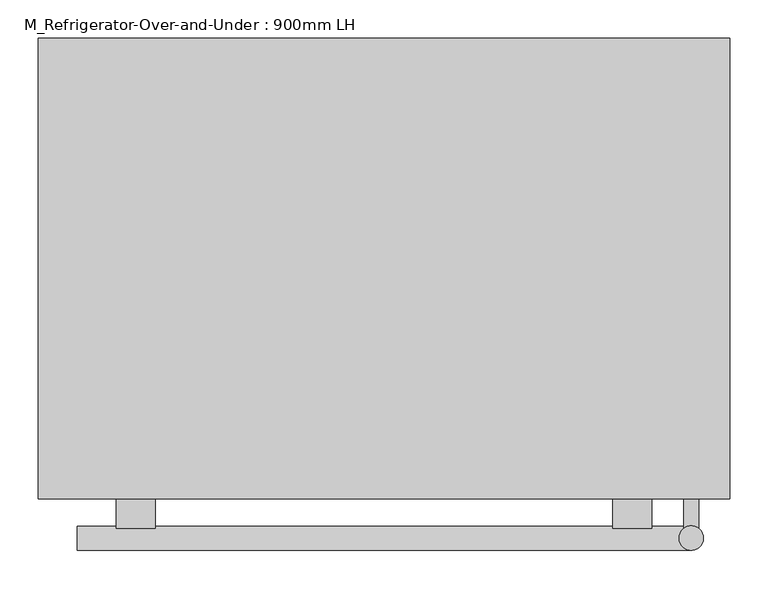
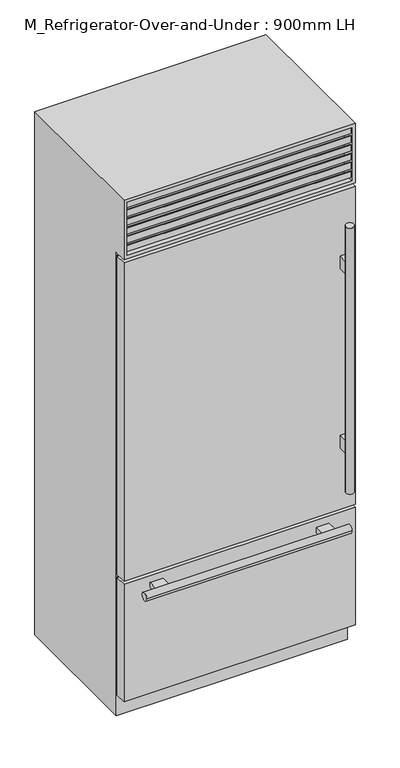
"""IFC4 building model written with IfcOpenShell, lengths in millimetres: proxy geometry, M_Refrigerator-Over-and-Under : 900mm LH."""

from ifc_helpers import new_model, si_unit, frame, origin, place, context, project, spatial, polyline, circle_curve, ellipse_curve, outline, extrude, faceted_brep, source, transform, mapped, element, save
from ifc_brep_helpers import plane_surface, cylinder_surface, advanced_brep


def m_refrigerator_over_and_under_900mm_lh_87200827(model_context):
    return source(origin(), model_context, "Body", "SolidModel", [
        extrude(outline(polyline([(-450.0, -655.55), (450.0, -655.55), (450.0, -700.0), (-450.0, -700.0), (-450.0, -655.55)])), frame((0.0, 0.0, 584.2), z_axis=(0.0, 0.0, 1.0), x_axis=(1.0, 0.0, 0.0)), (0.0, 0.0, 1.0), 1308.625),
        extrude(outline(polyline([(-450.0, -655.55), (450.0, -655.55), (450.0, -700.0), (-450.0, -700.0), (-450.0, -655.55)])), frame((0.0, 0.0, 88.9), z_axis=(0.0, 0.0, 1.0), x_axis=(1.0, 0.0, 0.0)), (0.0, 0.0, 1.0), 482.6),
        faceted_brep([(450.0, -700.0, 2150.0), (-450.0, -700.0, 2150.0), (-450.0, -700.0, 1905.525), (450.0, -700.0, 1905.525), (437.3, -700.0, 2137.3), (437.3, -700.0, 1918.225), (-437.3, -700.0, 1918.225), (-437.3, -700.0, 2137.3), (450.0, -100.0, 2150.0), (-450.0, -100.0, 2150.0), (-450.0, -100.0, 0.0), (-450.0, -649.2, 0.0), (-450.0, -649.2, 1905.525), (450.0, -649.2, 1905.525), (450.0, -649.2, 0.0), (450.0, -100.0, 0.0), (-437.3, -649.2, 2137.3), (437.3, -649.2, 2137.3), (-437.3, -649.2, 1918.225), (437.3, -649.2, 1918.225)], [[[0, 1, 2, 3], [4, 5, 6, 7]], [[1, 0, 8, 9]], [[2, 1, 9, 10, 11, 12]], [[3, 2, 12, 13]], [[8, 0, 3, 13, 14, 15]], [[4, 7, 16, 17]], [[7, 6, 18, 16]], [[6, 5, 19, 18]], [[5, 4, 17, 19]], [[15, 14, 11, 10]], [[9, 8, 15, 10]], [[17, 16, 18, 19]], [[11, 14, 13, 12]]]),
        extrude(outline(polyline([(-649.2, 1918.225), (-696.825, 1930.9860803), (-696.825, 1956.3860803), (-693.65, 1956.3860803), (-693.65, 1933.5368938), (-649.2, 1921.6265522), (-649.2, 1918.225)])), frame((-437.3, 0.0, 0.0), z_axis=(1.0, 0.0, 0.0), x_axis=(0.0, 1.0, 0.0)), (0.0, 0.0, 1.0), 874.6),
        extrude(outline(polyline([(-649.2, 1954.4077839), (-696.825, 1967.1688642), (-696.825, 1992.5688642), (-693.65, 1992.5688642), (-693.65, 1969.7196777), (-649.2, 1957.8093361), (-649.2, 1954.4077839)])), frame((-437.3, 0.0, 0.0), z_axis=(1.0, 0.0, 0.0), x_axis=(0.0, 1.0, 0.0)), (0.0, 0.0, 1.0), 874.6),
        extrude(outline(polyline([(-649.2, 1990.5905679), (-696.825, 2003.3516482), (-696.825, 2028.7516482), (-693.65, 2028.7516482), (-693.65, 2005.9024616), (-649.2, 1993.99212), (-649.2, 1990.5905679)])), frame((-437.3, 0.0, 0.0), z_axis=(1.0, 0.0, 0.0), x_axis=(0.0, 1.0, 0.0)), (0.0, 0.0, 1.0), 874.6),
        extrude(outline(polyline([(-649.2, 2026.7733518), (-696.825, 2039.5344321), (-696.825, 2064.9344321), (-693.65, 2064.9344321), (-693.65, 2042.0852456), (-649.2, 2030.174904), (-649.2, 2026.7733518)])), frame((-437.3, 0.0, 0.0), z_axis=(1.0, 0.0, 0.0), x_axis=(0.0, 1.0, 0.0)), (0.0, 0.0, 1.0), 874.6),
        extrude(outline(polyline([(-649.2, 2062.9561358), (-696.825, 2075.7172161), (-696.825, 2101.1172161), (-693.65, 2101.1172161), (-693.65, 2078.2680295), (-649.2, 2066.3576879), (-649.2, 2062.9561358)])), frame((-437.3, 0.0, 0.0), z_axis=(1.0, 0.0, 0.0), x_axis=(0.0, 1.0, 0.0)), (0.0, 0.0, 1.0), 874.6),
        extrude(outline(polyline([(-649.2, 2099.1389197), (-696.825, 2111.9), (-696.825, 2137.3), (-693.65, 2137.3), (-693.65, 2114.4508135), (-649.2, 2102.5404719), (-649.2, 2099.1389197)])), frame((-437.3, 0.0, 0.0), z_axis=(1.0, 0.0, 0.0), x_axis=(0.0, 1.0, 0.0)), (0.0, 0.0, 1.0), 874.6),
        advanced_brep(
        [(-443.65, -649.2, 565.15), (-443.65, -655.55, 565.15), (-443.65, -655.55, 95.25), (-443.65, -649.2, 95.25), (-446.825, -655.55, 568.325), (-446.825, -649.2, 568.325), (-446.825, -649.2, 92.075), (-446.825, -655.55, 92.075), (443.65, -655.55, 95.25), (443.65, -649.2, 95.25), (446.825, -649.2, 92.075), (446.825, -655.55, 92.075), (443.65, -655.55, 565.15), (443.65, -649.2, 565.15), (446.825, -649.2, 568.325), (446.825, -655.55, 568.325)],
        [
            (0, 1),
            (1, 2),
            (2, 3),
            (3, 0),
            (4, 5, ellipse_curve(frame((-446.825, -652.375, 568.325), z_axis=(-0.7071067811865475, 0.0, -0.7071067811865476), x_axis=(-0.7071067811865476, 0.0, 0.7071067811865475)), 4.4901281, 3.175)),
            (5, 6),
            (6, 7, ellipse_curve(frame((-446.825, -652.375, 92.075), z_axis=(-0.7071067811865475, 0.0, 0.7071067811865475), x_axis=(0.7071067811865474, 0.0, 0.7071067811865477)), 4.4901281, 3.175)),
            (7, 4),
            (2, 8),
            (8, 9),
            (9, 3),
            (6, 10),
            (10, 11, ellipse_curve(frame((446.825, -652.375, 92.075), z_axis=(-0.7071067811865475, 0.0, -0.7071067811865476), x_axis=(-0.7071067811865476, 0.0, 0.7071067811865474)), 4.4901281, 3.175)),
            (11, 7),
            (8, 12),
            (12, 13),
            (13, 9),
            (10, 14),
            (14, 15, ellipse_curve(frame((446.825, -652.375, 568.325), z_axis=(0.7071067811865476, 0.0, -0.7071067811865474), x_axis=(-0.7071067811865474, 0.0, -0.7071067811865477)), 4.4901281, 3.175)),
            (15, 11),
            (12, 1),
            (0, 13),
            (5, 14),
            (4, 15),
        ],
        [
            plane_surface(frame((-443.65, -655.55, 565.15), z_axis=(1.0, 0.0, 0.0), x_axis=(0.0, 0.0, -1.0))),
            cylinder_surface(frame((-446.825, -652.375, 571.5), z_axis=(0.0, 0.0, 1.0), x_axis=(0.0, -1.0, 0.0)), 3.175),
            plane_surface(frame((-443.65, -655.55, 95.25), z_axis=(0.0, 0.0, 1.0), x_axis=(1.0, 0.0, 0.0))),
            cylinder_surface(frame((-450.0, -652.375, 92.075), z_axis=(-1.0, 0.0, 0.0), x_axis=(0.0, -1.0, 0.0)), 3.175),
            plane_surface(frame((443.65, -655.55, 95.25), z_axis=(-1.0, 0.0, 0.0), x_axis=(0.0, 0.0, 1.0))),
            cylinder_surface(frame((446.825, -652.375, 88.9), z_axis=(0.0, 0.0, -1.0), x_axis=(0.0, -1.0, 0.0)), 3.175),
            plane_surface(frame((443.65, -655.55, 565.15), z_axis=(0.0, 0.0, -1.0), x_axis=(-1.0, 0.0, 0.0))),
            plane_surface(frame((443.65, -649.2, 565.15), z_axis=(0.0, 1.0, 0.0), x_axis=(-1.0, 0.0, 0.0))),
            cylinder_surface(frame((450.0, -652.375, 568.325), z_axis=(1.0, 0.0, 0.0), x_axis=(0.0, -1.0, 0.0)), 3.175),
            plane_surface(frame((446.825, -655.55, 568.325), z_axis=(0.0, -1.0, 0.0), x_axis=(-1.0, 0.0, 0.0))),
        ],
        [
            (0, [[1, 2, 3, 4]]),
            (1, [[5, 6, 7, 8]]),
            (2, [[-3, 9, 10, 11]]),
            (3, [[-7, 12, 13, 14]]),
            (4, [[-10, 15, 16, 17]]),
            (5, [[-13, 18, 19, 20]]),
            (6, [[-16, 21, -1, 22]]),
            (7, [[23, -18, -12, -6], [-11, -17, -22, -4]]),
            (8, [[-19, -23, -5, 24]]),
            (9, [[-14, -20, -24, -8], [-21, -15, -9, -2]]),
        ],
    ),
        advanced_brep(
        [(-443.65, -649.2, 1886.475), (-443.65, -655.55, 1886.475), (-443.65, -655.55, 590.55), (-443.65, -649.2, 590.55), (-446.825, -655.55, 1889.65), (-446.825, -649.2, 1889.65), (-446.825, -649.2, 587.375), (-446.825, -655.55, 587.375), (443.65, -655.55, 590.55), (443.65, -649.2, 590.55), (446.825, -649.2, 587.375), (446.825, -655.55, 587.375), (443.65, -655.55, 1886.475), (443.65, -649.2, 1886.475), (446.825, -649.2, 1889.65), (446.825, -655.55, 1889.65)],
        [
            (0, 1),
            (1, 2),
            (2, 3),
            (3, 0),
            (4, 5, ellipse_curve(frame((-446.825, -652.375, 1889.65), z_axis=(-0.7071067811865476, 0.0, -0.7071067811865475), x_axis=(-0.7071067811865475, 0.0, 0.7071067811865475)), 4.4901281, 3.175)),
            (5, 6),
            (6, 7, ellipse_curve(frame((-446.825, -652.375, 587.375), z_axis=(-0.7071067811865475, 0.0, 0.7071067811865476), x_axis=(0.7071067811865475, 0.0, 0.7071067811865475)), 4.4901281, 3.175)),
            (7, 4),
            (2, 8),
            (8, 9),
            (9, 3),
            (6, 10),
            (10, 11, ellipse_curve(frame((446.825, -652.375, 587.375), z_axis=(-0.7071067811865476, 0.0, -0.7071067811865475), x_axis=(-0.7071067811865475, 0.0, 0.7071067811865475)), 4.4901281, 3.175)),
            (11, 7),
            (8, 12),
            (12, 13),
            (13, 9),
            (10, 14),
            (14, 15, ellipse_curve(frame((446.825, -652.375, 1889.65), z_axis=(0.7071067811865474, 0.0, -0.7071067811865476), x_axis=(-0.7071067811865475, 0.0, -0.7071067811865476)), 4.4901281, 3.175)),
            (15, 11),
            (12, 1),
            (0, 13),
            (5, 14),
            (4, 15),
        ],
        [
            plane_surface(frame((-443.65, -655.55, 1886.475), z_axis=(1.0, 0.0, 0.0), x_axis=(0.0, 0.0, -1.0))),
            cylinder_surface(frame((-446.825, -652.375, 1892.825), z_axis=(0.0, 0.0, 1.0), x_axis=(0.0, -1.0, 0.0)), 3.175),
            plane_surface(frame((-443.65, -655.55, 590.55), z_axis=(0.0, 0.0, 1.0), x_axis=(1.0, 0.0, 0.0))),
            cylinder_surface(frame((-450.0, -652.375, 587.375), z_axis=(-1.0, 0.0, 0.0), x_axis=(0.0, -1.0, 0.0)), 3.175),
            plane_surface(frame((443.65, -655.55, 590.55), z_axis=(-1.0, 0.0, 0.0), x_axis=(0.0, 0.0, 1.0))),
            cylinder_surface(frame((446.825, -652.375, 584.2), z_axis=(0.0, 0.0, -1.0), x_axis=(0.0, -1.0, 0.0)), 3.175),
            plane_surface(frame((443.65, -655.55, 1886.475), z_axis=(0.0, 0.0, -1.0), x_axis=(-1.0, 0.0, 0.0))),
            plane_surface(frame((443.65, -649.2, 1886.475), z_axis=(0.0, 1.0, 0.0), x_axis=(-1.0, 0.0, 0.0))),
            cylinder_surface(frame((450.0, -652.375, 1889.65), z_axis=(1.0, 0.0, 0.0), x_axis=(0.0, -1.0, 0.0)), 3.175),
            plane_surface(frame((446.825, -655.55, 1889.65), z_axis=(0.0, -1.0, 0.0), x_axis=(-1.0, 0.0, 0.0))),
        ],
        [
            (0, [[1, 2, 3, 4]]),
            (1, [[5, 6, 7, 8]]),
            (2, [[-3, 9, 10, 11]]),
            (3, [[-7, 12, 13, 14]]),
            (4, [[-10, 15, 16, 17]]),
            (5, [[-13, 18, 19, 20]]),
            (6, [[-16, 21, -1, 22]]),
            (7, [[23, -18, -12, -6], [-11, -17, -22, -4]]),
            (8, [[-19, -23, -5, 24]]),
            (9, [[-14, -20, -24, -8], [-21, -15, -9, -2]]),
        ],
    ),
        advanced_brep(
        [(-297.6, -700.0, 542.925), (-297.6, -700.0, 523.875), (-348.4, -700.0, 523.875), (-348.4, -700.0, 542.925), (297.6, -700.0, 542.925), (348.4, -700.0, 542.925), (348.4, -700.0, 523.875), (297.6, -700.0, 523.875), (-297.6, -738.4741958, 542.925), (-297.6, -735.2991958, 533.4), (-297.6, -738.4741958, 523.875), (-348.4, -738.4741958, 523.875), (-348.4, -735.2991958, 533.4), (-348.4, -738.4741958, 542.925), (297.6, -738.4741958, 542.925), (348.4, -738.4741958, 542.925), (348.4, -735.2991958, 533.4), (348.4, -738.4741958, 523.875), (297.6, -738.4741958, 523.875), (297.6, -735.2991958, 533.4), (399.2, -767.0491958, 533.4), (399.2, -735.2991958, 533.4), (-399.2, -767.0491958, 533.4), (-399.2, -735.2991958, 533.4)],
        [
            (0, 1),
            (1, 2),
            (2, 3),
            (3, 0),
            (4, 5),
            (5, 6),
            (6, 7),
            (7, 4),
            (0, 8),
            (8, 9, circle_curve(frame((-297.6, -751.1741958, 533.4), z_axis=(-1.0, 0.0, 0.0), x_axis=(0.0, 1.0, 0.0)), 15.875)),
            (9, 10, circle_curve(frame((-297.6, -751.1741958, 533.4), z_axis=(-1.0, 0.0, 0.0), x_axis=(0.0, 1.0, 0.0)), 15.875)),
            (10, 1),
            (10, 11),
            (11, 2),
            (11, 12, circle_curve(frame((-348.4, -751.1741958, 533.4), z_axis=(1.0, 0.0, 0.0), x_axis=(0.0, 1.0, 0.0)), 15.875)),
            (12, 13, circle_curve(frame((-348.4, -751.1741958, 533.4), z_axis=(1.0, 0.0, 0.0), x_axis=(0.0, 1.0, 0.0)), 15.875)),
            (13, 3),
            (13, 8),
            (4, 14),
            (14, 15),
            (15, 5),
            (15, 16, circle_curve(frame((348.4, -751.1741958, 533.4), z_axis=(-1.0, 0.0, 0.0), x_axis=(0.0, 1.0, 0.0)), 15.875)),
            (16, 17, circle_curve(frame((348.4, -751.1741958, 533.4), z_axis=(-1.0, 0.0, 0.0), x_axis=(0.0, 1.0, 0.0)), 15.875)),
            (17, 6),
            (17, 18),
            (18, 7),
            (18, 19, circle_curve(frame((297.6, -751.1741958, 533.4), z_axis=(1.0, 0.0, 0.0), x_axis=(0.0, 1.0, 0.0)), 15.875)),
            (19, 14, circle_curve(frame((297.6, -751.1741958, 533.4), z_axis=(1.0, 0.0, 0.0), x_axis=(0.0, 1.0, 0.0)), 15.875)),
            (20, 21, circle_curve(frame((399.2, -751.1741958, 533.4), z_axis=(1.0, 0.0, 0.0), x_axis=(0.0, 1.0, 0.0)), 15.875)),
            (21, 20, circle_curve(frame((399.2, -751.1741958, 533.4), z_axis=(1.0, 0.0, 0.0), x_axis=(0.0, 1.0, 0.0)), 15.875)),
            (22, 23, circle_curve(frame((-399.2, -751.1741958, 533.4), z_axis=(-1.0, 0.0, 0.0), x_axis=(0.0, 1.0, 0.0)), 15.875)),
            (23, 22, circle_curve(frame((-399.2, -751.1741958, 533.4), z_axis=(-1.0, 0.0, 0.0), x_axis=(0.0, 1.0, 0.0)), 15.875)),
            (20, 22),
            (23, 12),
            (9, 19),
            (16, 21),
        ],
        [
            plane_surface(frame((-297.6, -700.0, 542.925), z_axis=(0.0, 1.0, 0.0), x_axis=(0.0, 0.0, -1.0))),
            plane_surface(frame((-297.6, -700.0, 542.925), z_axis=(1.0, 0.0, 0.0), x_axis=(0.0, -1.0, 0.0))),
            plane_surface(frame((-297.6, -700.0, 523.875), z_axis=(0.0, 0.0, -1.0), x_axis=(0.0, -1.0, 0.0))),
            plane_surface(frame((-348.4, -700.0, 523.875), z_axis=(-1.0, 0.0, 0.0), x_axis=(0.0, -1.0, 0.0))),
            plane_surface(frame((-348.4, -700.0, 542.925), z_axis=(0.0, 0.0, 1.0), x_axis=(0.0, -1.0, 0.0))),
            plane_surface(frame((297.6, -700.0, 542.925), z_axis=(0.0, 0.0, 1.0), x_axis=(0.0, -1.0, 0.0))),
            plane_surface(frame((348.4, -700.0, 542.925), z_axis=(1.0, 0.0, 0.0), x_axis=(0.0, -1.0, 0.0))),
            plane_surface(frame((348.4, -700.0, 523.875), z_axis=(0.0, 0.0, -1.0), x_axis=(0.0, -1.0, 0.0))),
            plane_surface(frame((297.6, -700.0, 523.875), z_axis=(-1.0, 0.0, 0.0), x_axis=(0.0, -1.0, 0.0))),
            plane_surface(frame((399.2, -735.2991958, 533.4), z_axis=(1.0, 0.0, 0.0), x_axis=(0.0, 0.0, 1.0))),
            plane_surface(frame((-399.2, -735.2991958, 533.4), z_axis=(-1.0, 0.0, 0.0), x_axis=(0.0, 0.0, -1.0))),
            cylinder_surface(frame((-399.2, -751.1741958, 533.4), z_axis=(1.0, 0.0, 0.0), x_axis=(0.0, 1.0, 0.0)), 15.875),
        ],
        [
            (0, [[1, 2, 3, 4]]),
            (0, [[5, 6, 7, 8]]),
            (1, [[-1, 9, 10, 11, 12]]),
            (2, [[-2, -12, 13, 14]]),
            (3, [[-3, -14, 15, 16, 17]]),
            (4, [[-4, -17, 18, -9]]),
            (5, [[-5, 19, 20, 21]]),
            (6, [[-6, -21, 22, 23, 24]]),
            (7, [[-7, -24, 25, 26]]),
            (8, [[-8, -26, 27, 28, -19]]),
            (9, [[29, 30]]),
            (10, [[31, 32]]),
            (11, [[-29, 33, -32, 34, -15, -13, -11, 35, -27, -25, -23, 36]]),
            (11, [[-30, -36, -22, -20, -28, -35, -10, -18, -16, -34, -31, -33]]),
        ],
    ),
        advanced_brep(
        [(409.525, -700.0, 1626.125), (409.525, -700.0, 1575.325), (390.475, -700.0, 1575.325), (390.475, -700.0, 1626.125), (409.525, -700.0, 889.0), (409.525, -700.0, 838.2), (390.475, -700.0, 838.2), (390.475, -700.0, 889.0), (409.525, -738.4741958, 1626.125), (409.525, -738.4741958, 1575.325), (390.475, -738.4741958, 1575.325), (390.475, -738.4741958, 1626.125), (409.525, -738.4741958, 889.0), (409.525, -738.4741958, 838.2), (390.475, -738.4741958, 838.2), (390.475, -738.4741958, 889.0), (384.125, -751.1741958, 1778.525), (415.875, -751.1741958, 1778.525), (384.125, -751.1741958, 685.8), (415.875, -751.1741958, 685.8)],
        [
            (0, 1),
            (1, 2),
            (2, 3),
            (3, 0),
            (4, 5),
            (5, 6),
            (6, 7),
            (7, 4),
            (0, 8),
            (8, 9),
            (9, 1),
            (9, 10, circle_curve(frame((400.0, -751.1741958, 1575.325), z_axis=(0.0, 0.0, 1.0), x_axis=(1.0, 0.0, 0.0)), 15.875)),
            (10, 2),
            (10, 11),
            (11, 3),
            (11, 8, circle_curve(frame((400.0, -751.1741958, 1626.125), z_axis=(0.0, 0.0, -1.0), x_axis=(1.0, 0.0, 0.0)), 15.875)),
            (4, 12),
            (12, 13),
            (13, 5),
            (13, 14, circle_curve(frame((400.0, -751.1741958, 838.2), z_axis=(0.0, 0.0, 1.0), x_axis=(1.0, 0.0, 0.0)), 15.875)),
            (14, 6),
            (14, 15),
            (15, 7),
            (15, 12, circle_curve(frame((400.0, -751.1741958, 889.0), z_axis=(0.0, 0.0, -1.0), x_axis=(1.0, 0.0, 0.0)), 15.875)),
            (16, 17, circle_curve(frame((400.0, -751.1741958, 1778.525), z_axis=(0.0, 0.0, 1.0), x_axis=(1.0, 0.0, 0.0)), 15.875)),
            (17, 16, circle_curve(frame((400.0, -751.1741958, 1778.525), z_axis=(0.0, 0.0, 1.0), x_axis=(1.0, 0.0, 0.0)), 15.875)),
            (18, 19, circle_curve(frame((400.0, -751.1741958, 685.8), z_axis=(0.0, 0.0, -1.0), x_axis=(1.0, 0.0, 0.0)), 15.875)),
            (19, 18, circle_curve(frame((400.0, -751.1741958, 685.8), z_axis=(0.0, 0.0, -1.0), x_axis=(1.0, 0.0, 0.0)), 15.875)),
            (16, 18),
            (19, 17),
        ],
        [
            plane_surface(frame((409.525, -700.0, 1626.125), z_axis=(0.0, 1.0, 0.0), x_axis=(0.0, 0.0, -1.0))),
            plane_surface(frame((409.525, -700.0, 1626.125), z_axis=(1.0, 0.0, 0.0), x_axis=(0.0, -1.0, 0.0))),
            plane_surface(frame((409.525, -700.0, 1575.325), z_axis=(0.0, 0.0, -1.0), x_axis=(0.0, -1.0, 0.0))),
            plane_surface(frame((390.475, -700.0, 1575.325), z_axis=(-1.0, 0.0, 0.0), x_axis=(0.0, -1.0, 0.0))),
            plane_surface(frame((390.475, -700.0, 1626.125), z_axis=(0.0, 0.0, 1.0), x_axis=(0.0, -1.0, 0.0))),
            plane_surface(frame((409.525, -700.0, 889.0), z_axis=(1.0, 0.0, 0.0), x_axis=(0.0, -1.0, 0.0))),
            plane_surface(frame((409.525, -700.0, 838.2), z_axis=(0.0, 0.0, -1.0), x_axis=(0.0, -1.0, 0.0))),
            plane_surface(frame((390.475, -700.0, 838.2), z_axis=(-1.0, 0.0, 0.0), x_axis=(0.0, -1.0, 0.0))),
            plane_surface(frame((390.475, -700.0, 889.0), z_axis=(0.0, 0.0, 1.0), x_axis=(0.0, -1.0, 0.0))),
            plane_surface(frame((415.875, -751.1741958, 1778.525), z_axis=(0.0, 0.0, 1.0), x_axis=(0.0, 1.0, 0.0))),
            plane_surface(frame((415.875, -751.1741958, 685.8), z_axis=(0.0, 0.0, -1.0), x_axis=(0.0, -1.0, 0.0))),
            cylinder_surface(frame((400.0, -751.1741958, 685.8), z_axis=(0.0, 0.0, 1.0), x_axis=(1.0, 0.0, 0.0)), 15.875),
        ],
        [
            (0, [[1, 2, 3, 4]]),
            (0, [[5, 6, 7, 8]]),
            (1, [[-1, 9, 10, 11]]),
            (2, [[-2, -11, 12, 13]]),
            (3, [[-3, -13, 14, 15]]),
            (4, [[-4, -15, 16, -9]]),
            (5, [[-5, 17, 18, 19]]),
            (6, [[-6, -19, 20, 21]]),
            (7, [[-7, -21, 22, 23]]),
            (8, [[-8, -23, 24, -17]]),
            (9, [[25, 26]]),
            (10, [[27, 28]]),
            (11, [[-25, 29, -28, 30]]),
            (11, [[-26, -30, -27, -29], [-10, -16, -14, -12], [-18, -24, -22, -20]]),
        ],
    ),
    ])


if __name__ == "__main__":
    model = new_model("IFC4")
    model_context = context("Model", 3, world=origin())
    ifc_project = project(units=[si_unit("LENGTHUNIT", "METRE", prefix="MILLI")], contexts=[model_context])
    site = spatial("IfcSite", under=ifc_project)
    building = spatial("IfcBuilding", under=site)
    placement = place(None, origin())
    m_refrigerator_over_and_under_900mm_lh_shape = m_refrigerator_over_and_under_900mm_lh_87200827(model_context)
    element("IfcBuildingElementProxy", 1, Name="M_Refrigerator-Over-and-Under : 900mm LH", ObjectType="M_Refrigerator-Over-and-Under : 900mm LH", at=placement, inside=building, context=model_context, shape_type="MappedRepresentation", body=[
        mapped(m_refrigerator_over_and_under_900mm_lh_shape, transform((0.0, 0.0, 0.0), x_axis=(1.0, 0.0, 0.0), y_axis=(0.0, 1.0, 0.0), z_axis=(0.0, 0.0, 1.0))),
    ])
    save(model, "model.ifc")

# Revit data of these elements
# Type "M_Refrigerator-Over-and-Under : 900mm LH"
#   Label = ""
#   Description = "Over-and-Under Refrigerator"
#   Assembly Code = "E1090320"
#   Width = 0.9 m
#   Wall Offset = 0.1 m
#   Voltage = 120 V
#   Power Consumption = 1000 VA
#   Height = 2.15 m
#   Handle Centerline = 0.85 m
#   Depth = 0.6 m
#   Amperage = 8.33333 A
#   Show Label = no
#   RH = no
#   LH = yes
#   Gasket = Appliance - Gasket
#   Appliance Finish = Appliance - Gasket
# Element 1 (IfcBuildingElementProxy, "M_Refrigerator-Over-and-Under : 900mm LH")
#   Materials on its faces: "Appliance - Gasket"
# Materials
#   "Appliance - Gasket": class "Miscellaneous", colour RGB 234 234 234, transparency 0, Cost = 0
